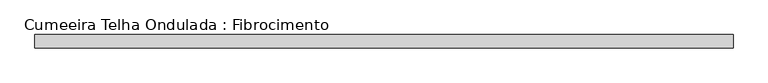
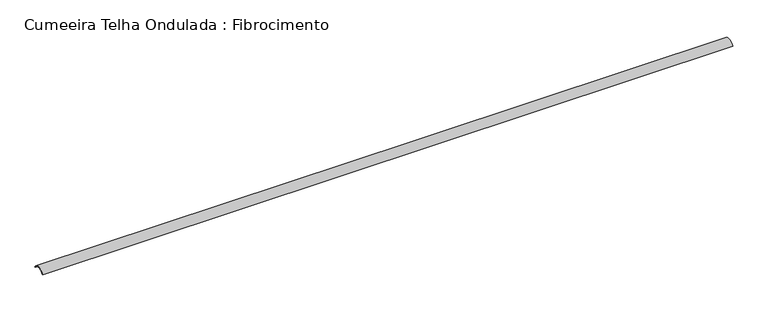
"""IFC4 building model written with IfcOpenShell, lengths in millimetres: beam geometry, Cumeeira Telha Ondulada : Fibrocimento."""

from ifc_helpers import new_model, si_unit, point, frame, frame_2d, origin, place, context, project, spatial, polyline, circle_curve, trimmed, segment, composite_curve, outline, extrude, source, transform, mapped, element, save


def cumeeira_telha_ondulada_fibrocimento_e54732c7(model_context):
    return source(origin(), model_context, "Body", "SweptSolid", [
        extrude(outline(composite_curve([segment(polyline([(58.3970135, 42.4437972), (53.9055884, 40.2467307)]), True, "CONTINUOUS"), segment(trimmed(circle_curve(frame_2d((-1.6029865, 13.0936483)), 61.7939461), [point((53.9055884, 40.2467307))], [point((-57.1115615, 40.2467307))], True, "CARTESIAN"), True, "CONTINUOUS"), segment(polyline([(-57.1115615, 40.2467307), (-61.6029865, 42.4437972)]), True, "CONTINUOUS"), segment(trimmed(circle_curve(frame_2d((-1.6029865, 13.0936483)), 66.7939461), [point((-61.6029865, 42.4437972))], [point((58.3970135, 42.4437972))], False, "CARTESIAN"), True, "CONTINUOUS")], self_intersect=False)), frame((-3133.4781794, 0.0, 0.0), z_axis=(1.0, 0.0, 0.0), x_axis=(0.0, 1.0, 0.0)), (0.0, 0.0, 1.0), 6266.9563589),
    ])


if __name__ == "__main__":
    model = new_model("IFC4")
    model_context = context("Model", 3, world=origin())
    ifc_project = project(units=[si_unit("LENGTHUNIT", "METRE", prefix="MILLI")], contexts=[model_context])
    site = spatial("IfcSite", under=ifc_project)
    building = spatial("IfcBuilding", under=site)
    placement = place(None, origin())
    cumeeira_telha_ondulada_fibrocimento_shape = cumeeira_telha_ondulada_fibrocimento_e54732c7(model_context)
    element("IfcBeam", 1, ObjectType="Cumeeira Telha Ondulada : Fibrocimento", at=placement, inside=building, context=model_context, shape_type="MappedRepresentation", body=[
        mapped(cumeeira_telha_ondulada_fibrocimento_shape, transform((0.0, 0.0, 0.0), x_axis=(1.0, 0.0, 0.0), y_axis=(0.0, 1.0, 0.0), z_axis=(0.0, 0.0, 1.0))),
    ])
    save(model, "model.ifc")

# Revit data of these elements
# Type "Cumeeira Telha Ondulada : Fibrocimento"
#   Cost = 5
#   Length [instance default] = 1.524 m
#   b = 0.07 m
#   h = 0.16 m
#   Structural Material = .TELHA DE FIBROCIMENTO
#   Assembly Code = ""
# Element 1 (IfcBeam, "Cumeeira Telha Ondulada : Fibrocimento")
#   Materials on its faces: ".TELHA DE FIBROCIMENTO"
# Materials
#   ".TELHA DE FIBROCIMENTO": class "CC_TELHADO", colour RGB 77 77 76, transparency 0, Description = "TELHA ONDULADA FIBROCIMENTO", Cost = 0
